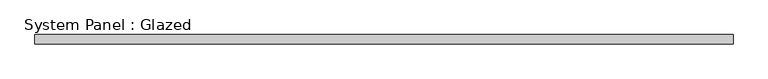
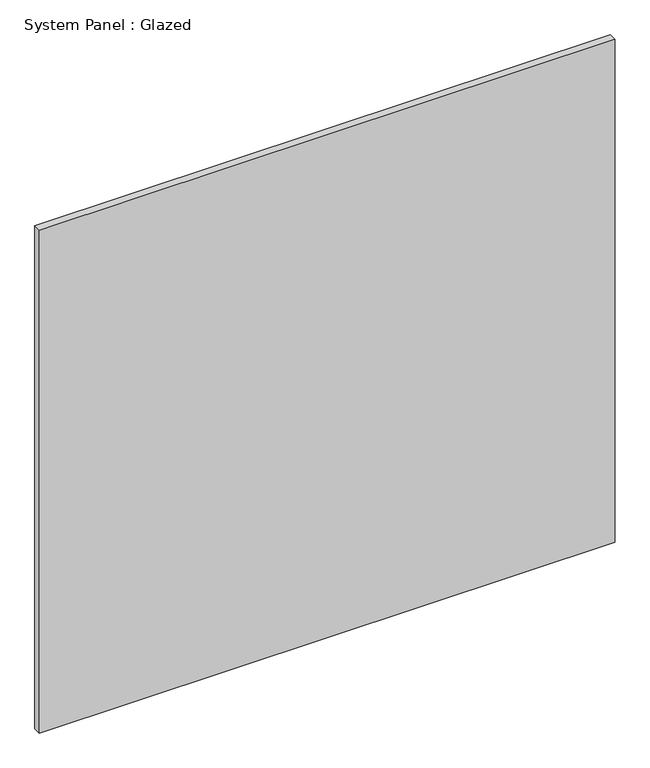
"""IFC4 building model written with IfcOpenShell, lengths in millimetres: plate geometry, System Panel : Glazed."""

from ifc_helpers import new_model, si_unit, origin, origin_with_axes, place, context, project, spatial, polyline, outline, extrude, source, transform, mapped, element, save


def system_panel_glazed_359e611f(model_context):
    return source(origin(), model_context, "Body", "SweptSolid", [
        extrude(outline(polyline([(915.0000002, 24.5), (-915.0000002, 24.5), (-915.0000002, 49.5), (915.0000002, 49.5), (915.0000002, 24.5)])), origin_with_axes(), (0.0, 0.0, 1.0), 1690.2939092),
    ])


if __name__ == "__main__":
    model = new_model("IFC4")
    model_context = context("Model", 3, world=origin())
    ifc_project = project(units=[si_unit("LENGTHUNIT", "METRE", prefix="MILLI")], contexts=[model_context])
    site = spatial("IfcSite", under=ifc_project)
    building = spatial("IfcBuilding", under=site)
    placement = place(None, origin())
    system_panel_glazed_shape = system_panel_glazed_359e611f(model_context)
    element("IfcPlate", 1, ObjectType="System Panel : Glazed", at=placement, inside=building, context=model_context, shape_type="MappedRepresentation", body=[
        mapped(system_panel_glazed_shape, transform((0.0, 0.0, 0.0), x_axis=(1.0, 0.0, 0.0), y_axis=(0.0, 1.0, 0.0), z_axis=(0.0, 0.0, 1.0))),
    ])
    save(model, "model.ifc")

# Revit data of these elements
# Element 1 (IfcPlate, "System Panel : Glazed")
#   Materials on its faces: "Glass"
# Materials
#   "Glass": class "Glass", colour RGB 218 227 224, transparency 0.85, Description = "Soda Lime Glass", Cost = 0
